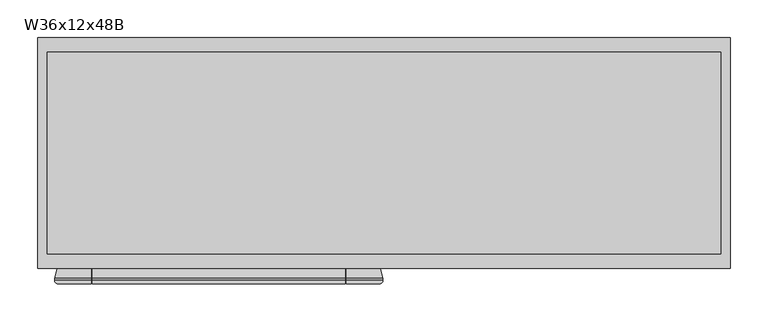
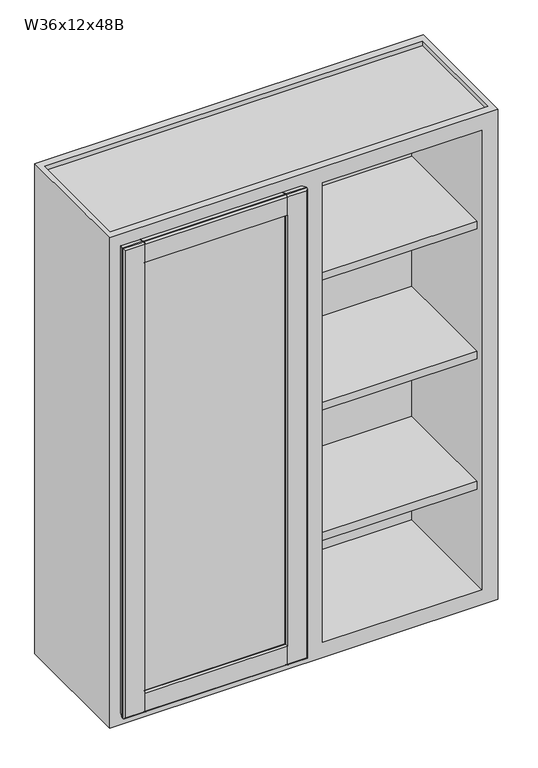
"""IFC4 building model written with IfcOpenShell, lengths in millimetres: furniture geometry, Cabinet-Wall-Merillat-Double_Door-Marlin : W36x12x48B."""

from ifc_helpers import new_model, si_unit, frame, origin, place, context, project, spatial, polyline, circle_curve, ellipse_curve, outline, extrude, faceted_brep, source, transform, mapped, element, save
from ifc_brep_helpers import plane_surface, cylinder_surface, advanced_brep


def w36x12x48b_7f092fba(model_context):
    return source(origin(), model_context, "Body", "SolidModel", [
        advanced_brep(
        [(-328.8971608, -401.6121, 2108.2), (-328.8971608, -401.6121, 939.8), (-325.8006683, -406.0825, 942.8964925), (-325.8006683, -406.0825, 2105.1035075), (-328.8971608, -398.8435, 2108.2), (-328.8971608, -398.8435, 939.8), (-325.3919608, -385.7625, 2104.6948), (-325.3919608, -385.7625, 943.3052), (-280.695998, -385.7625, 2059.9988372), (-280.3258663, -386.55625, 2059.6287055), (-278.2447073, -391.01931, 2057.5475465), (-278.2447073, -391.01931, 990.4524535), (-280.3258663, -386.55625, 988.3712945), (-280.695998, -385.7625, 988.0011628), (-279.6444767, -393.2594093, 2058.947316), (-279.6444767, -393.2594093, 989.052684), (-293.9721608, -393.5095, 2073.275), (-293.9721608, -393.5095, 974.725), (-293.9721608, -398.3355, 2073.275), (-293.9721608, -398.3355, 974.725), (-279.6444767, -398.5855907, 2058.947316), (-279.6444767, -398.5855907, 989.052684), (-278.2447073, -400.82569, 2057.5475465), (-278.2447073, -400.82569, 990.4524535), (-280.3258663, -405.28875, 2059.6287055), (-280.6931306, -406.0763508, 2059.9959698), (-280.695998, -406.0825, 988.0011628), (-280.3258663, -405.28875, 988.3712945), (101.3938467, -406.0825, 942.8964925), (56.3261206, -406.0825, 942.8964925), (56.3261206, -401.6121, 939.8), (104.4903392, -401.6121, 939.8), (-280.6931306, -401.6121, 939.8), (-280.6931306, -406.0825, 942.8964925), (-279.1056306, -401.6121, 939.8), (54.7386206, -401.6121, 939.8), (54.7386206, -406.0825, 942.8964925), (-279.1056306, -406.0825, 942.8964925), (56.3261206, -398.8435, 939.8), (104.4903392, -398.8435, 939.8), (-280.6931306, -398.8435, 939.8), (-279.1056306, -398.8435, 939.8), (54.7386206, -398.8435, 939.8), (56.3261206, -385.7625, 943.3052), (100.9851392, -385.7625, 943.3052), (-280.6931306, -385.7625, 943.3052), (-279.1056306, -385.7625, 943.3052), (54.7386206, -385.7625, 943.3052), (53.8378857, -391.01931, 990.4524535), (55.9190448, -386.55625, 988.3712945), (54.7386206, -386.55625, 988.3712945), (54.7386206, -385.7625, 988.0011628), (-279.1056306, -385.7625, 988.0011628), (-279.1056306, -386.55625, 988.3712945), (55.2376552, -393.2594093, 989.052684), (69.5653392, -393.5095, 974.725), (69.5653392, -398.3355, 974.725), (55.2376552, -398.5855907, 989.052684), (53.8378857, -400.82569, 990.4524535), (-279.1056306, -405.28875, 988.3712945), (-279.1056306, -406.0825, 988.0011628), (54.7386206, -406.0825, 988.0011628), (54.7386206, -405.28875, 988.3712945), (55.9190448, -405.28875, 988.3712945), (104.4903392, -401.6121, 2108.2), (101.3938467, -406.0825, 2105.1035075), (104.4903392, -398.8435, 2108.2), (100.9851392, -385.7625, 2104.6948), (56.2891765, -385.7625, 988.0011628), (53.8378857, -391.01931, 2057.5475465), (55.9190448, -386.55625, 2059.6287055), (56.2891765, -385.7625, 2059.9988372), (55.2376552, -393.2594093, 2058.947316), (69.5653392, -393.5095, 2073.275), (69.5653392, -398.3355, 2073.275), (55.2376552, -398.5855907, 2058.947316), (53.8378857, -400.82569, 2057.5475465), (56.2891765, -406.0825, 988.0011628), (56.2891765, -406.0825, 2059.9988372), (55.9190448, -405.28875, 2059.6287055), (-280.6931306, -406.0825, 2105.1035075), (-280.6931306, -401.6121, 2108.2), (56.3261206, -401.6121, 2108.2), (56.3261206, -406.0825, 2105.1035075), (54.7386206, -401.6121, 2108.2), (-279.1056306, -401.6121, 2108.2), (-279.1056306, -406.0825, 2105.1035075), (54.7386206, -406.0825, 2105.1035075), (-280.6931306, -398.8435, 2108.2), (56.3261206, -398.8435, 2108.2), (54.7386206, -398.8435, 2108.2), (-279.1056306, -398.8435, 2108.2), (-280.6931306, -385.7625, 2104.6948), (56.3261206, -385.7625, 2104.6948), (54.7386206, -385.7625, 2104.6948), (-279.1056306, -385.7625, 2104.6948), (54.7386206, -385.7625, 2059.9988372), (-279.1056306, -385.7625, 2059.9988372), (-279.1056306, -386.55625, 2059.6287055), (54.7386206, -386.55625, 2059.6287055), (54.7386206, -405.28875, 2059.6287055), (54.7386206, -406.0825, 2059.9988372), (-279.1056306, -406.0825, 2059.9988372), (-279.1056306, -405.28875, 2059.6287055), (54.7386206, -405.28875, 2104.9526052), (54.7386206, -401.6121, 2107.40625), (54.7386206, -398.9480037, 2107.40625), (54.7386206, -386.55625, 2104.0857412), (56.3261206, -386.55625, 2059.6287055), (56.3261206, -386.55625, 2104.0857412), (56.3261206, -398.9480037, 2107.40625), (56.3261206, -401.6121, 2107.40625), (56.3261206, -405.28875, 2104.9526052), (56.3261206, -405.28875, 2059.6287055), (-280.6931306, -405.28875, 2059.6287055), (-280.6931306, -405.28875, 2104.9526052), (-280.6931306, -401.6121, 2107.40625), (-280.6931306, -398.9480037, 2107.40625), (-280.6931306, -386.55625, 2104.0857412), (-280.6931306, -386.55625, 2059.6287055), (-279.1056306, -386.55625, 2104.0857412), (-279.1056306, -398.9480037, 2107.40625), (-279.1056306, -401.6121, 2107.40625), (-279.1056306, -405.28875, 2104.9526052), (-280.6931306, -386.55625, 988.3712945), (-280.6931306, -386.55625, 943.9142588), (-280.6931306, -398.9480037, 940.59375), (-280.6931306, -401.6121, 940.59375), (-280.6931306, -405.28875, 943.0473948), (-280.6931306, -405.28875, 988.3712945), (-279.1056306, -405.28875, 943.0473948), (-279.1056306, -401.6121, 940.59375), (-279.1056306, -398.9480037, 940.59375), (-279.1056306, -386.55625, 943.9142588), (54.7386206, -386.55625, 943.9142588), (54.7386206, -398.9480037, 940.59375), (54.7386206, -401.6121, 940.59375), (54.7386206, -405.28875, 943.0473948), (56.3261206, -405.28875, 988.3712945), (56.3261206, -405.28875, 943.0473948), (56.3261206, -401.6121, 940.59375), (56.3261206, -398.9480037, 940.59375), (56.3261206, -386.55625, 943.9142588), (56.3261206, -386.55625, 988.3712945)],
        [
            (0, 1),
            (1, 2, ellipse_curve(frame((-324.1219608, -401.6121, 944.5752), z_axis=(-0.7071067811865475, 0.0, 0.7071067811865475), x_axis=(0.7071067811865474, 0.0, 0.7071067811865476)), 6.7531526, 4.7752)),
            (2, 3),
            (3, 0, ellipse_curve(frame((-324.1219608, -401.6121, 2103.4248), z_axis=(-0.7071067811865475, 0.0, -0.7071067811865475), x_axis=(-0.7071067811865474, 0.0, 0.7071067811865476)), 6.7531526, 4.7752)),
            (0, 4),
            (4, 5),
            (5, 1),
            (4, 6),
            (6, 7),
            (7, 5),
            (8, 9),
            (9, 10),
            (10, 11),
            (11, 12),
            (12, 13),
            (13, 8),
            (10, 14, ellipse_curve(frame((-279.6719608, -391.6848492, 2058.9748), z_axis=(-0.7071067811865475, 0.0, -0.7071067811865475), x_axis=(-0.7071067811865474, 0.0, 0.7071067811865476)), 2.2271035, 1.5748)),
            (14, 15),
            (15, 11, ellipse_curve(frame((-279.6719608, -391.6848492, 989.0252), z_axis=(-0.7071067811865475, 0.0, 0.7071067811865475), x_axis=(0.7071067811865474, 0.0, 0.7071067811865476)), 2.2271035, 1.5748)),
            (14, 16),
            (16, 17),
            (17, 15),
            (16, 18),
            (18, 19),
            (19, 17),
            (18, 20),
            (20, 21),
            (21, 19),
            (20, 22, ellipse_curve(frame((-279.6719608, -400.1601508, 2058.9748), z_axis=(-0.7071067811865475, 0.0, -0.7071067811865475), x_axis=(-0.7071067811865474, 0.0, 0.7071067811865476)), 2.2271035, 1.5748)),
            (22, 23),
            (23, 21, ellipse_curve(frame((-279.6719608, -400.1601508, 989.0252), z_axis=(-0.7071067811865475, 0.0, 0.7071067811865475), x_axis=(0.7071067811865474, 0.0, 0.7071067811865476)), 2.2271035, 1.5748)),
            (22, 24),
            (24, 25),
            (25, 26),
            (26, 27),
            (27, 23),
            (28, 29),
            (29, 30, circle_curve(frame((56.3261206, -401.6121, 944.5752), z_axis=(1.0, 0.0, 0.0), x_axis=(0.0, 1.0, 0.0)), 4.7752)),
            (30, 31),
            (31, 28, ellipse_curve(frame((99.7151392, -401.6121, 944.5752), z_axis=(-0.7071067811865475, 0.0, -0.7071067811865475), x_axis=(-0.7071067811865476, 0.0, 0.7071067811865474)), 6.7531526, 4.7752)),
            (1, 32),
            (32, 33, circle_curve(frame((-280.6931306, -401.6121, 944.5752), z_axis=(-1.0, 0.0, 0.0), x_axis=(0.0, 1.0, 0.0)), 4.7752)),
            (33, 2),
            (34, 35),
            (35, 36, circle_curve(frame((54.7386206, -401.6121, 944.5752), z_axis=(-1.0, 0.0, 0.0), x_axis=(0.0, 1.0, 0.0)), 4.7752)),
            (36, 37),
            (37, 34, circle_curve(frame((-279.1056306, -401.6121, 944.5752), z_axis=(1.0, 0.0, 0.0), x_axis=(0.0, 1.0, 0.0)), 4.7752)),
            (30, 38),
            (38, 39),
            (39, 31),
            (5, 40),
            (40, 32),
            (41, 42),
            (42, 35),
            (34, 41),
            (38, 43),
            (43, 44),
            (44, 39),
            (7, 45),
            (45, 40),
            (46, 47),
            (47, 42),
            (41, 46),
            (48, 49),
            (49, 50),
            (50, 51),
            (51, 52),
            (52, 53),
            (53, 12),
            (11, 48),
            (15, 54),
            (54, 48, ellipse_curve(frame((55.2651392, -391.6848492, 989.0252), z_axis=(-0.7071067811865475, 0.0, -0.7071067811865475), x_axis=(-0.7071067811865476, 0.0, 0.7071067811865474)), 2.2271035, 1.5748)),
            (17, 55),
            (55, 54),
            (19, 56),
            (56, 55),
            (21, 57),
            (57, 56),
            (23, 58),
            (58, 57, ellipse_curve(frame((55.2651392, -400.1601508, 989.0252), z_axis=(-0.7071067811865475, 0.0, -0.7071067811865475), x_axis=(-0.7071067811865476, 0.0, 0.7071067811865474)), 2.2271035, 1.5748)),
            (27, 59),
            (59, 60),
            (60, 61),
            (61, 62),
            (62, 63),
            (63, 58),
            (31, 64),
            (64, 65, ellipse_curve(frame((99.7151392, -401.6121, 2103.4248), z_axis=(0.7071067811865475, 0.0, -0.7071067811865475), x_axis=(-0.7071067811865474, 0.0, -0.7071067811865476)), 6.7531526, 4.7752)),
            (65, 28),
            (39, 66),
            (66, 64),
            (44, 67),
            (67, 66),
            (68, 49),
            (48, 69),
            (69, 70),
            (70, 71),
            (71, 68),
            (54, 72),
            (72, 69, ellipse_curve(frame((55.2651392, -391.6848492, 2058.9748), z_axis=(0.7071067811865475, 0.0, -0.7071067811865475), x_axis=(-0.7071067811865474, 0.0, -0.7071067811865476)), 2.2271035, 1.5748)),
            (55, 73),
            (73, 72),
            (56, 74),
            (74, 73),
            (57, 75),
            (75, 74),
            (58, 76),
            (76, 75, ellipse_curve(frame((55.2651392, -400.1601508, 2058.9748), z_axis=(0.7071067811865475, 0.0, -0.7071067811865475), x_axis=(-0.7071067811865474, 0.0, -0.7071067811865476)), 2.2271035, 1.5748)),
            (63, 77),
            (77, 78),
            (78, 79),
            (79, 76),
            (3, 80),
            (80, 81, circle_curve(frame((-280.6931306, -401.6121, 2103.4248), z_axis=(-1.0, 0.0, 0.0), x_axis=(0.0, 1.0, 0.0)), 4.7752)),
            (81, 0),
            (64, 82),
            (82, 83, circle_curve(frame((56.3261206, -401.6121, 2103.4248), z_axis=(1.0, 0.0, 0.0), x_axis=(0.0, 1.0, 0.0)), 4.7752)),
            (83, 65),
            (84, 85),
            (85, 86, circle_curve(frame((-279.1056306, -401.6121, 2103.4248), z_axis=(1.0, 0.0, 0.0), x_axis=(0.0, 1.0, 0.0)), 4.7752)),
            (86, 87),
            (87, 84, circle_curve(frame((54.7386206, -401.6121, 2103.4248), z_axis=(-1.0, 0.0, 0.0), x_axis=(0.0, 1.0, 0.0)), 4.7752)),
            (81, 88),
            (88, 4),
            (66, 89),
            (89, 82),
            (90, 91),
            (91, 85),
            (84, 90),
            (88, 92),
            (92, 6),
            (67, 93),
            (93, 89),
            (94, 95),
            (95, 91),
            (90, 94),
            (51, 47),
            (46, 52),
            (92, 8),
            (13, 45),
            (43, 68),
            (71, 93),
            (96, 97),
            (97, 95),
            (94, 96),
            (9, 98),
            (98, 97),
            (96, 99),
            (99, 70),
            (69, 10),
            (72, 14),
            (73, 16),
            (74, 18),
            (75, 20),
            (76, 22),
            (79, 100),
            (100, 101),
            (101, 102),
            (102, 103),
            (103, 24),
            (33, 26),
            (25, 80),
            (36, 61),
            (60, 37),
            (83, 78),
            (77, 29),
            (86, 102),
            (101, 87),
            (100, 104),
            (104, 105, circle_curve(frame((54.7386206, -401.6121, 2103.4248), z_axis=(-1.0, 0.0, 0.0), x_axis=(0.0, 0.0, 1.0)), 3.98145)),
            (105, 106),
            (106, 107),
            (107, 99),
            (71, 108),
            (108, 109),
            (109, 110),
            (110, 111),
            (111, 112, circle_curve(frame((56.3261206, -401.6121, 2103.4248), z_axis=(1.0, 0.0, 0.0), x_axis=(0.0, 0.0, 1.0)), 3.98145)),
            (112, 113),
            (113, 78),
            (113, 79),
            (112, 104),
            (111, 105),
            (110, 106),
            (109, 107),
            (108, 70),
            (25, 114),
            (114, 115),
            (115, 116, circle_curve(frame((-280.6931306, -401.6121, 2103.4248), z_axis=(-1.0, 0.0, 0.0), x_axis=(0.0, 0.0, 1.0)), 3.98145)),
            (116, 117),
            (117, 118),
            (118, 119),
            (119, 8),
            (98, 120),
            (120, 121),
            (121, 122),
            (122, 123, circle_curve(frame((-279.1056306, -401.6121, 2103.4248), z_axis=(1.0, 0.0, 0.0), x_axis=(0.0, 0.0, 1.0)), 3.98145)),
            (123, 103),
            (24, 114),
            (123, 115),
            (122, 116),
            (121, 117),
            (120, 118),
            (9, 119),
            (13, 124),
            (124, 125),
            (125, 126),
            (126, 127),
            (127, 128, circle_curve(frame((-280.6931306, -401.6121, 944.5752), z_axis=(-1.0, 0.0, 0.0), x_axis=(0.0, 0.0, 1.0)), 3.98145)),
            (128, 129),
            (129, 26),
            (59, 130),
            (130, 131, circle_curve(frame((-279.1056306, -401.6121, 944.5752), z_axis=(1.0, 0.0, 0.0), x_axis=(0.0, 0.0, 1.0)), 3.98145)),
            (131, 132),
            (132, 133),
            (133, 53),
            (12, 124),
            (133, 125),
            (132, 126),
            (131, 127),
            (130, 128),
            (27, 129),
            (50, 134),
            (134, 135),
            (135, 136),
            (136, 137, circle_curve(frame((54.7386206, -401.6121, 944.5752), z_axis=(-1.0, 0.0, 0.0), x_axis=(0.0, 0.0, 1.0)), 3.98145)),
            (137, 62),
            (138, 139),
            (139, 140, circle_curve(frame((56.3261206, -401.6121, 944.5752), z_axis=(1.0, 0.0, 0.0), x_axis=(0.0, 0.0, 1.0)), 3.98145)),
            (140, 141),
            (141, 142),
            (142, 143),
            (143, 68),
            (77, 138),
            (63, 138),
            (143, 49),
            (142, 134),
            (141, 135),
            (140, 136),
            (139, 137),
        ],
        [
            cylinder_surface(frame((-324.1219608, -401.6121, 2108.2), z_axis=(0.0, 0.0, 1.0), x_axis=(0.0, 1.0, 0.0)), 4.7752),
            plane_surface(frame((-328.8971608, -401.6121, 2108.2), z_axis=(-1.0, 0.0, 0.0), x_axis=(0.0, 0.0, -1.0))),
            plane_surface(frame((-328.8971608, -398.8435, 2108.2), z_axis=(-0.9659229350723619, 0.25882983502910506, 0.0), x_axis=(0.0, 0.0, -1.0))),
            plane_surface(frame((-280.695998, -385.7625, 2059.9988372), z_axis=(0.9063077870366099, 0.4226182617407856, 0.0), x_axis=(0.0, 0.0, -1.0))),
            cylinder_surface(frame((-279.6719608, -391.6848492, 2108.2), z_axis=(0.0, 0.0, 1.0000000000000002), x_axis=(0.01745240643729364, -0.9998476951563912, 0.0)), 1.5748),
            plane_surface(frame((-279.6444767, -393.2594093, 2058.947316), z_axis=(0.017452406437322144, -0.9998476951563906, 0.0), x_axis=(0.0, 0.0, -1.0))),
            plane_surface(frame((-293.9721608, -393.5095, 2073.275), z_axis=(1.0, 0.0, 0.0), x_axis=(0.0, 0.0, -1.0))),
            plane_surface(frame((-293.9721608, -398.3355, 2073.275), z_axis=(0.01745240643727848, 0.9998476951563914, 0.0), x_axis=(0.0, 0.0, -1.0))),
            cylinder_surface(frame((-279.6719608, -400.1601508, 2108.2), z_axis=(0.0, 0.0, 1.0000000000000002), x_axis=(0.9063077870367326, -0.42261826174052236, 0.0)), 1.5748),
            plane_surface(frame((-278.2447073, -400.82569, 2057.5475465), z_axis=(0.9063077870366333, -0.4226182617407352, 0.0), x_axis=(0.0, 0.0, -1.0))),
            cylinder_surface(frame((-328.8971608, -401.6121, 944.5752), z_axis=(-1.0, 0.0, 0.0), x_axis=(0.0, 1.0, 0.0)), 4.7752),
            plane_surface(frame((-328.8971608, -401.6121, 939.8), z_axis=(0.0, 0.0, -1.0), x_axis=(1.0, 0.0, 0.0))),
            plane_surface(frame((-328.8971608, -398.8435, 939.8), z_axis=(0.0, 0.2588298350291095, -0.9659229350723607), x_axis=(1.0, 0.0, 0.0))),
            plane_surface(frame((-280.695998, -385.7625, 988.0011628), z_axis=(0.0, 0.42261826174078143, 0.9063077870366119), x_axis=(1.0, 0.0, 0.0))),
            cylinder_surface(frame((-328.8971608, -391.6848492, 989.0252), z_axis=(-1.0000000000000002, 0.0, 0.0), x_axis=(0.0, -0.9998476951563913, 0.017452406437289025)), 1.5748),
            plane_surface(frame((-279.6444767, -393.2594093, 989.052684), z_axis=(0.0, -0.9998476951563907, 0.01745240643731753), x_axis=(1.0, 0.0, 0.0))),
            plane_surface(frame((-293.9721608, -393.5095, 974.725), z_axis=(0.0, 0.0, 1.0), x_axis=(1.0, 0.0, 0.0))),
            plane_surface(frame((-293.9721608, -398.3355, 974.725), z_axis=(0.0, 0.9998476951563913, 0.017452406437283095), x_axis=(1.0, 0.0, 0.0))),
            cylinder_surface(frame((-328.8971608, -400.1601508, 989.0252), z_axis=(-1.0000000000000002, 0.0, 0.0), x_axis=(0.0, -0.4226182617405265, 0.9063077870367306)), 1.5748),
            plane_surface(frame((-278.2447073, -400.82569, 990.4524535), z_axis=(0.0, -0.4226182617407394, 0.9063077870366314), x_axis=(1.0, 0.0, 0.0))),
            cylinder_surface(frame((99.7151392, -401.6121, 939.8), z_axis=(0.0, 0.0, -1.0), x_axis=(0.0, 1.0, 0.0)), 4.7752),
            plane_surface(frame((104.4903392, -401.6121, 939.8), z_axis=(1.0, 0.0, 0.0), x_axis=(0.0, 0.0, 1.0))),
            plane_surface(frame((104.4903392, -398.8435, 939.8), z_axis=(0.9659229350723619, 0.25882983502910506, 0.0), x_axis=(0.0, 0.0, 1.0))),
            plane_surface(frame((56.2891765, -385.7625, 988.0011628), z_axis=(-0.9063077870366099, 0.4226182617407856, 0.0), x_axis=(0.0, 0.0, 1.0))),
            cylinder_surface(frame((55.2651392, -391.6848492, 939.8), z_axis=(0.0, 0.0, -1.0000000000000002), x_axis=(-0.01745240643729364, -0.9998476951563912, 0.0)), 1.5748),
            plane_surface(frame((55.2376552, -393.2594093, 989.052684), z_axis=(-0.017452406437322144, -0.9998476951563906, 0.0), x_axis=(0.0, 0.0, 1.0))),
            plane_surface(frame((69.5653392, -393.5095, 974.725), z_axis=(-1.0, 0.0, 0.0), x_axis=(0.0, 0.0, 1.0))),
            plane_surface(frame((69.5653392, -398.3355, 974.725), z_axis=(-0.01745240643727848, 0.9998476951563914, 0.0), x_axis=(0.0, 0.0, 1.0))),
            cylinder_surface(frame((55.2651392, -400.1601508, 939.8), z_axis=(0.0, 0.0, -1.0000000000000002), x_axis=(-0.9063077870367326, -0.42261826174052236, 0.0)), 1.5748),
            plane_surface(frame((53.8378857, -400.82569, 990.4524535), z_axis=(-0.9063077870366333, -0.4226182617407352, 0.0), x_axis=(0.0, 0.0, 1.0))),
            cylinder_surface(frame((104.4903392, -401.6121, 2103.4248), z_axis=(1.0, 0.0, 0.0), x_axis=(0.0, 1.0, 0.0)), 4.7752),
            plane_surface(frame((104.4903392, -401.6121, 2108.2), z_axis=(0.0, 0.0, 1.0), x_axis=(-1.0, 0.0, 0.0))),
            plane_surface(frame((104.4903392, -398.8435, 2108.2), z_axis=(0.0, 0.2588298350291006, 0.9659229350723632), x_axis=(-1.0, 0.0, 0.0))),
            plane_surface(frame((100.9851392, -385.7625, 2104.6948), z_axis=(0.0, 1.0, 0.0), x_axis=(-1.0, 0.0, 0.0))),
            plane_surface(frame((56.2891765, -385.7625, 2059.9988372), z_axis=(0.0, 0.42261826174078976, -0.9063077870366079), x_axis=(-1.0, 0.0, 0.0))),
            cylinder_surface(frame((104.4903392, -391.6848492, 2058.9748), z_axis=(1.0000000000000002, 0.0, 0.0), x_axis=(0.0, -0.999847695156391, -0.017452406437298253)), 1.5748),
            plane_surface(frame((55.2376552, -393.2594093, 2058.947316), z_axis=(0.0, -0.9998476951563905, -0.01745240643732676), x_axis=(-1.0, 0.0, 0.0))),
            plane_surface(frame((69.5653392, -393.5095, 2073.275), z_axis=(0.0, 0.0, -1.0), x_axis=(-1.0, 0.0, 0.0))),
            plane_surface(frame((69.5653392, -398.3355, 2073.275), z_axis=(0.0, 0.9998476951563915, -0.017452406437273867), x_axis=(-1.0, 0.0, 0.0))),
            cylinder_surface(frame((104.4903392, -400.1601508, 2058.9748), z_axis=(1.0000000000000002, 0.0, 0.0), x_axis=(0.0, -0.4226182617405182, -0.9063077870367346)), 1.5748),
            plane_surface(frame((53.8378857, -400.82569, 2057.5475465), z_axis=(0.0, -0.422618261740731, -0.9063077870366353), x_axis=(-1.0, 0.0, 0.0))),
            plane_surface(frame((56.2891765, -406.0825, 2059.9988372), z_axis=(0.0, -1.0, 0.0), x_axis=(-1.0, 0.0, 0.0))),
            plane_surface(frame((54.7386206, -406.0825, 2059.9988372), z_axis=(1.0000000000000002, 0.0, 0.0), x_axis=(0.0, 0.906307787036639, -0.4226182617407233))),
            plane_surface(frame((56.3261206, -406.0825, 2059.9988372), z_axis=(-1.0000000000000002, 0.0, 0.0), x_axis=(0.0, -0.906307787036639, 0.4226182617407233))),
            plane_surface(frame((54.7386206, -406.0825, 2059.9988372), z_axis=(0.0, 0.4226182617407233, 0.906307787036639), x_axis=(1.0, 0.0, 0.0))),
            plane_surface(frame((54.7386206, -405.28875, 2059.6287055), z_axis=(0.0, -1.0, 0.0), x_axis=(1.0, 0.0, 0.0))),
            cylinder_surface(frame((56.3261206, -401.6121, 2103.4248), z_axis=(1.0, 0.0, 0.0), x_axis=(0.0, 0.0, 1.0)), 3.98145),
            plane_surface(frame((54.7386206, -401.6121, 2107.40625), z_axis=(0.0, 0.0, 1.0), x_axis=(1.0, 0.0, 0.0))),
            plane_surface(frame((54.7386206, -398.9480037, 2107.40625), z_axis=(0.0, 0.25882983502917667, 0.9659229350723427), x_axis=(1.0, 0.0, 0.0))),
            plane_surface(frame((54.7386206, -386.55625, 2104.0857412), z_axis=(0.0, 1.0, 0.0), x_axis=(1.0, 0.0, 0.0))),
            plane_surface(frame((54.7386206, -386.55625, 2059.6287055), z_axis=(0.0, -0.4226182617408151, 0.906307787036596), x_axis=(1.0, 0.0, 0.0))),
            plane_surface(frame((-280.6931306, -406.0825, 2059.9988372), z_axis=(1.0000000000000002, 0.0, 0.0), x_axis=(0.0, 0.9063077870366527, -0.4226182617406937))),
            plane_surface(frame((-279.1056306, -406.0825, 2059.9988372), z_axis=(-1.0000000000000002, 0.0, 0.0), x_axis=(0.0, -0.9063077870366527, 0.4226182617406937))),
            plane_surface(frame((-280.6931306, -406.0825, 2059.9988372), z_axis=(0.0, 0.4226182617406937, 0.9063077870366527), x_axis=(1.0, 0.0, 0.0))),
            plane_surface(frame((-280.6931306, -405.28875, 2059.6287055), z_axis=(0.0, -1.0, 0.0), x_axis=(1.0, 0.0, 0.0))),
            cylinder_surface(frame((-279.1056306, -401.6121, 2103.4248), z_axis=(1.0, 0.0, 0.0), x_axis=(0.0, 0.0, 1.0)), 3.98145),
            plane_surface(frame((-280.6931306, -401.6121, 2107.40625), z_axis=(0.0, 0.0, 1.0), x_axis=(1.0, 0.0, 0.0))),
            plane_surface(frame((-280.6931306, -398.9480037, 2107.40625), z_axis=(0.0, 0.25882983502917556, 0.9659229350723431), x_axis=(1.0, 0.0, 0.0))),
            plane_surface(frame((-280.6931306, -386.55625, 2104.0857412), z_axis=(0.0, 1.0, 0.0), x_axis=(1.0, 0.0, 0.0))),
            plane_surface(frame((-280.6931306, -386.55625, 2059.6287055), z_axis=(0.0, -0.4226182617408452, 0.906307787036582), x_axis=(1.0, 0.0, 0.0))),
            plane_surface(frame((-280.6931306, -401.6121, 949.3504), z_axis=(1.0, 0.0, 0.0), x_axis=(0.0, -1.0, 0.0))),
            plane_surface(frame((-279.1056306, -401.6121, 949.3504), z_axis=(-1.0, 0.0, 0.0), x_axis=(0.0, 1.0, 0.0))),
            plane_surface(frame((-280.6931306, -385.7625, 988.0011628), z_axis=(0.0, -0.4226182617407559, -0.9063077870366237), x_axis=(1.0, 0.0, 0.0))),
            plane_surface(frame((-280.6931306, -386.55625, 988.3712945), z_axis=(0.0, 1.0, 0.0), x_axis=(1.0, 0.0, 0.0))),
            plane_surface(frame((-280.6931306, -386.55625, 943.9142588), z_axis=(0.0, 0.2588298350294462, -0.9659229350722706), x_axis=(1.0, 0.0, 0.0))),
            plane_surface(frame((-280.6931306, -398.9480037, 940.59375), z_axis=(0.0, 0.0, -1.0), x_axis=(1.0, 0.0, 0.0))),
            cylinder_surface(frame((-279.1056306, -401.6121, 944.5752), z_axis=(1.0, 0.0, 0.0), x_axis=(0.0, 0.0, 1.0)), 3.98145),
            plane_surface(frame((-280.6931306, -405.28875, 943.0473948), z_axis=(0.0, -1.0, 0.0), x_axis=(1.0, 0.0, 0.0))),
            plane_surface(frame((-280.6931306, -405.28875, 988.3712945), z_axis=(0.0, 0.4226182617407407, -0.9063077870366308), x_axis=(1.0, 0.0, 0.0))),
            plane_surface(frame((54.7386206, -405.28875, 988.3712945), z_axis=(1.0000000000000002, 0.0, 0.0), x_axis=(0.0, -0.906307787036642, -0.42261826174071665))),
            plane_surface(frame((56.3261206, -405.28875, 988.3712945), z_axis=(-1.0000000000000002, 0.0, 0.0), x_axis=(0.0, 0.906307787036642, 0.42261826174071665))),
            plane_surface(frame((54.7386206, -405.28875, 988.3712945), z_axis=(0.0, 0.42261826174071665, -0.906307787036642), x_axis=(1.0, 0.0, 0.0))),
            plane_surface(frame((54.7386206, -385.7625, 988.0011628), z_axis=(0.0, -0.42261826174079165, -0.9063077870366071), x_axis=(1.0, 0.0, 0.0))),
            plane_surface(frame((54.7386206, -386.55625, 988.3712945), z_axis=(0.0, 1.0, 0.0), x_axis=(1.0, 0.0, 0.0))),
            plane_surface(frame((54.7386206, -386.55625, 943.9142588), z_axis=(0.0, 0.2588298350294473, -0.9659229350722702), x_axis=(1.0, 0.0, 0.0))),
            plane_surface(frame((54.7386206, -398.9480037, 940.59375), z_axis=(0.0, 0.0, -1.0), x_axis=(1.0, 0.0, 0.0))),
            cylinder_surface(frame((56.3261206, -401.6121, 944.5752), z_axis=(1.0, 0.0, 0.0), x_axis=(0.0, 0.0, 1.0)), 3.98145),
            plane_surface(frame((54.7386206, -405.28875, 943.0473948), z_axis=(0.0, -1.0, 0.0), x_axis=(1.0, 0.0, 0.0))),
        ],
        [
            (0, [[1, 2, 3, 4]]),
            (1, [[5, 6, 7, -1]]),
            (2, [[8, 9, 10, -6]]),
            (3, [[11, 12, 13, 14, 15, 16]]),
            (4, [[17, 18, 19, -13]]),
            (5, [[20, 21, 22, -18]]),
            (6, [[23, 24, 25, -21]]),
            (7, [[26, 27, 28, -24]]),
            (8, [[29, 30, 31, -27]]),
            (9, [[32, 33, 34, 35, 36, -30]]),
            (10, [[37, 38, 39, 40]]),
            (10, [[41, 42, 43, -2]]),
            (10, [[44, 45, 46, 47]]),
            (11, [[-39, 48, 49, 50]]),
            (11, [[51, 52, -41, -7]]),
            (11, [[53, 54, -44, 55]]),
            (12, [[-49, 56, 57, 58]]),
            (12, [[59, 60, -51, -10]]),
            (12, [[61, 62, -53, 63]]),
            (13, [[64, 65, 66, 67, 68, 69, -14, 70]]),
            (14, [[71, 72, -70, -19]]),
            (15, [[73, 74, -71, -22]]),
            (16, [[75, 76, -73, -25]]),
            (17, [[77, 78, -75, -28]]),
            (18, [[79, 80, -77, -31]]),
            (19, [[-36, 81, 82, 83, 84, 85, 86, -79]]),
            (20, [[87, 88, 89, -40]]),
            (21, [[90, 91, -87, -50]]),
            (22, [[92, 93, -90, -58]]),
            (23, [[94, -64, 95, 96, 97, 98]]),
            (24, [[99, 100, -95, -72]]),
            (25, [[101, 102, -99, -74]]),
            (26, [[103, 104, -101, -76]]),
            (27, [[105, 106, -103, -78]]),
            (28, [[107, 108, -105, -80]]),
            (29, [[-86, 109, 110, 111, 112, -107]]),
            (30, [[113, 114, 115, -4]]),
            (30, [[116, 117, 118, -88]]),
            (30, [[119, 120, 121, 122]]),
            (31, [[-115, 123, 124, -5]]),
            (31, [[125, 126, -116, -91]]),
            (31, [[127, 128, -119, 129]]),
            (32, [[-124, 130, 131, -8]]),
            (32, [[132, 133, -125, -93]]),
            (32, [[134, 135, -127, 136]]),
            (33, [[-67, 137, -61, 138]]),
            (33, [[-131, 139, -16, 140, -59, -9]]),
            (33, [[-57, 141, -98, 142, -132, -92]]),
            (33, [[143, 144, -134, 145]]),
            (34, [[-12, 146, 147, -143, 148, 149, -96, 150]]),
            (35, [[-150, -100, 151, -17]]),
            (36, [[-151, -102, 152, -20]]),
            (37, [[-152, -104, 153, -23]]),
            (38, [[-153, -106, 154, -26]]),
            (39, [[-154, -108, 155, -29]]),
            (40, [[-112, 156, 157, 158, 159, 160, -32, -155]]),
            (41, [[-43, 161, -34, 162, -113, -3]]),
            (41, [[-46, 163, -83, 164]]),
            (41, [[-118, 165, -110, 166, -37, -89]]),
            (41, [[-121, 167, -158, 168]]),
            (42, [[-148, -145, -136, -129, -122, -168, -157, 169, 170, 171, 172, 173]]),
            (43, [[-165, -117, -126, -133, -142, 174, 175, 176, 177, 178, 179, 180]]),
            (44, [[181, -111, -180]]),
            (45, [[-156, -181, -179, 182, -169]]),
            (46, [[-182, -178, 183, -170]]),
            (47, [[-183, -177, 184, -171]]),
            (48, [[-184, -176, 185, -172]]),
            (49, [[-185, -175, 186, -149, -173]]),
            (50, [[-97, -186, -174]]),
            (51, [[-139, -130, -123, -114, -162, 187, 188, 189, 190, 191, 192, 193]]),
            (52, [[-159, -167, -120, -128, -135, -144, -147, 194, 195, 196, 197, 198]]),
            (53, [[-33, 199, -187]]),
            (54, [[-199, -160, -198, 200, -188]]),
            (55, [[-200, -197, 201, -189]]),
            (56, [[-201, -196, 202, -190]]),
            (57, [[-202, -195, 203, -191]]),
            (58, [[-203, -194, -146, 204, -192]]),
            (59, [[-204, -11, -193]]),
            (60, [[-161, -42, -52, -60, -140, 205, 206, 207, 208, 209, 210, 211]]),
            (61, [[-68, -138, -63, -55, -47, -164, -82, 212, 213, 214, 215, 216]]),
            (62, [[-15, 217, -205]]),
            (63, [[-217, -69, -216, 218, -206]]),
            (64, [[-218, -215, 219, -207]]),
            (65, [[-219, -214, 220, -208]]),
            (66, [[-220, -213, 221, -209]]),
            (67, [[-221, -212, -81, 222, -210]]),
            (68, [[-222, -35, -211]]),
            (69, [[-84, -163, -45, -54, -62, -137, -66, 223, 224, 225, 226, 227]]),
            (70, [[228, 229, 230, 231, 232, 233, -141, -56, -48, -38, -166, 234]]),
            (71, [[-109, 235, -234]]),
            (72, [[236, -94, -233]]),
            (73, [[-65, -236, -232, 237, -223]]),
            (74, [[-237, -231, 238, -224]]),
            (75, [[-238, -230, 239, -225]]),
            (76, [[-239, -229, 240, -226]]),
            (77, [[-240, -228, -235, -85, -227]]),
        ],
    ),
        extrude(outline(polyline([(69.5653392, -398.3355), (-293.9721608, -398.3355), (-293.9721608, -393.5095), (69.5653392, -393.5095), (69.5653392, -398.3355)])), frame((0.0, 0.0, 974.725), z_axis=(0.0, 0.0, 1.0), x_axis=(1.0, 0.0, 0.0)), (0.0, 0.0, 1.0), 1098.55),
        extrude(outline(polyline([(-313.3711577, -366.7125), (-313.3711577, -100.0125), (525.0128185, -100.0125), (525.0128185, -366.7125), (-313.3711577, -366.7125)])), frame((0.0, 0.0, 1838.325), z_axis=(0.0, 0.0, 1.0), x_axis=(1.0, 0.0, 0.0)), (0.0, 0.0, 1.0), 19.05),
        extrude(outline(polyline([(-313.3711577, -366.7125), (-313.3711577, -100.0125), (525.0128185, -100.0125), (525.0128185, -366.7125), (-313.3711577, -366.7125)])), frame((0.0, 0.0, 1190.625), z_axis=(0.0, 0.0, 1.0), x_axis=(1.0, 0.0, 0.0)), (0.0, 0.0, 1.0), 19.05),
        extrude(outline(polyline([(-313.3711577, -366.7125), (-313.3711577, -100.0125), (525.0128185, -100.0125), (525.0128185, -366.7125), (-313.3711577, -366.7125)])), frame((0.0, 0.0, 1514.475), z_axis=(0.0, 0.0, 1.0), x_axis=(1.0, 0.0, 0.0)), (0.0, 0.0, 1.0), 19.05),
        faceted_brep([(-351.1221608, -80.9625, 2133.6), (563.2778392, -80.9625, 2133.6), (563.2778392, -80.9625, 914.4), (-351.1221608, -80.9625, 914.4), (-351.1221608, -385.7625, 2133.6), (-351.1221608, -385.7625, 914.4), (563.2778392, -385.7625, 914.4), (563.2778392, -385.7625, 2133.6), (525.0128185, -385.7625, 2095.2735163), (525.0128185, -385.7625, 952.2672696), (149.5690685, -385.7625, 952.2672696), (149.5690685, -385.7625, 2095.2735163), (-313.3711577, -385.7625, 2095.2735163), (62.58661, -385.7625, 2095.2735163), (62.58661, -385.7625, 952.2672696), (-313.3711577, -385.7625, 952.2672696), (-338.4221608, -100.0125, 914.4), (-338.4221608, -366.7125, 914.4), (550.5778392, -366.7125, 914.4), (550.5778392, -100.0125, 914.4), (550.5778392, -366.7125, 2133.6), (-338.4221608, -366.7125, 2133.6), (-338.4221608, -100.0125, 2133.6), (550.5778392, -100.0125, 2133.6), (-313.3711577, -100.0125, 2095.2735163), (525.0128185, -100.0125, 2095.2735163), (149.5690685, -366.7125, 2095.2735163), (62.58661, -366.7125, 2095.2735163), (525.0128185, -100.0125, 952.2672696), (-313.3711577, -100.0125, 952.2672696), (62.58661, -366.7125, 952.2672696), (149.5690685, -366.7125, 952.2672696), (550.5778392, -100.0125, 2122.9851371), (-338.4221608, -100.0125, 2122.9851371), (-338.4221608, -366.7125, 2122.9851371), (550.5778392, -366.7125, 2122.9851371), (-338.4221608, -100.0125, 924.2352657), (550.5778392, -100.0125, 924.2352657), (550.5778392, -366.7125, 924.2352657), (-338.4221608, -366.7125, 924.2352657)], [[[0, 1, 2, 3]], [[4, 5, 6, 7], [8, 9, 10, 11], [12, 13, 14, 15]], [[3, 5, 4, 0]], [[2, 6, 5, 3], [16, 17, 18, 19]], [[1, 7, 6, 2]], [[0, 4, 7, 1], [20, 21, 22, 23]], [[24, 25, 8, 11, 26, 27, 13, 12]], [[8, 25, 28, 9]], [[28, 29, 15, 14, 30, 31, 10, 9]], [[15, 29, 24, 12]], [[32, 33, 34, 35]], [[35, 20, 23, 32]], [[34, 21, 20, 35]], [[33, 22, 21, 34]], [[32, 23, 22, 33]], [[36, 37, 38, 39]], [[36, 16, 19, 37]], [[37, 19, 18, 38]], [[38, 18, 17, 39]], [[39, 17, 16, 36]], [[24, 29, 28, 25]], [[26, 11, 10, 31]], [[13, 27, 30, 14]], [[31, 30, 27, 26]]]),
    ])


if __name__ == "__main__":
    model = new_model("IFC4")
    model_context = context("Model", 3, world=origin())
    ifc_project = project(units=[si_unit("LENGTHUNIT", "METRE", prefix="MILLI")], contexts=[model_context])
    site = spatial("IfcSite", under=ifc_project)
    building = spatial("IfcBuilding", under=site)
    placement = place(None, origin())
    w36x12x48b_shape = w36x12x48b_7f092fba(model_context)
    element("IfcFurniture", 1, ObjectType="Cabinet-Wall-Merillat-Double_Door-Marlin : W36x12x48B", at=placement, inside=building, context=model_context, shape_type="MappedRepresentation", body=[
        mapped(w36x12x48b_shape, transform((0.0, 0.0, 0.0), x_axis=(1.0, 0.0, 0.0), y_axis=(0.0, 1.0, 0.0), z_axis=(0.0, 0.0, 1.0))),
    ])
    save(model, "model.ifc")

# Revit data of these elements
# Type "Cabinet-Wall-Merillat-Double_Door-Marlin : W36x12x48B"
#   URL = "https://www.merillat.com/"
#   Product Page URL = "https://www.merillat.com/our-products/"
#   Product Line = "Express"
#   Product Group = "Wall Cabinet"
#   Product Documentation Link = "http://merillatbusiness.com/wp-content/uploads/2014/07/Merillat_Classic_Catalog.pdf"
#   Model = "W3642B"
#   Manufacturer = "Merillat"
#   Height Note = "Actual Height of 21 inches Cabinet is 20 1/2 inches"
#   Glass Door Note = "Glass Cabinet doors are only available in specific sizes. Please refer to the catalog for this information before requesting a glass size."
#   Finish = "Wood"
#   Description = "Wall 3642 Butt Door"
#   Construction Type = "Wall Cabinet"
#   Cabinet Construction Note = "Cabinets with B suffix have BUTT doors without a center frame stile:"
#   Assembly Code = "C1030410"
#   Spacing = 0' - 1"
#   Shelving Height = 0' - 11 1/4"
#   Door Spacing = 0' - 0 1/8"
#   Cabinet Door Width = 1' - 5 1/16"
#   Cabinet Door Height = 3' - 10"
#   Depth = 1' - 0"
#   Height = 4' - 0"
#   Top Of Cabinet = 7' - 0"
#   Width = 3' - 0"
#   COBie.Type = no
#   Top and Bottom Visibility = yes
#   Partial Overlay Butt = yes
#   Partial Overlay = no
#   Number of Shelves Greater than one = 3
#   Number of Shelves = 3
#   Middle Shelf = yes
#   Full Overlay Butt = no
#   Full Overlay = no
#   Elevation Swing Line = yes
#   Door Drawer Material = Wood - Merillat - Pecan(1)
#   Cabinet Material = Wood - Merillat - Pecan(1)
#   Cabinet Door Style = element 806847
# Element 1 (IfcFurniture, "Cabinet-Wall-Merillat-Double_Door-Marlin : W36x12x48B")
#   Materials on its faces: "Wood - Merillat - Pecan(1)"
# Materials
#   "Wood - Merillat - Pecan(1)": class "Wood", colour RGB 108 67 43, transparency 0, Cost = 0
